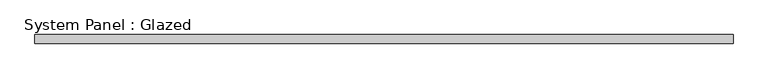
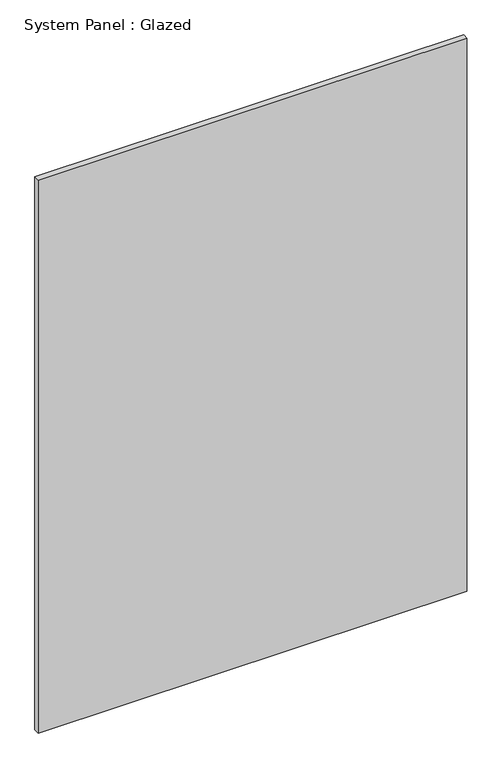
"""IFC4 building model written with IfcOpenShell, lengths in millimetres: plate geometry, System Panel : Glazed."""

from ifc_helpers import new_model, si_unit, origin, origin_with_axes, place, context, project, spatial, polyline, outline, extrude, source, transform, mapped, element, save


def system_panel_glazed_43d21894(model_context):
    return source(origin(), model_context, "Body", "SweptSolid", [
        extrude(outline(polyline([(962.5000001, 24.5), (-962.5000001, 24.5), (-962.5000001, 49.5), (962.5000001, 49.5), (962.5000001, 24.5)])), origin_with_axes(), (0.0, 0.0, 1.0), 2625.0),
    ])


if __name__ == "__main__":
    model = new_model("IFC4")
    model_context = context("Model", 3, world=origin())
    ifc_project = project(units=[si_unit("LENGTHUNIT", "METRE", prefix="MILLI")], contexts=[model_context])
    site = spatial("IfcSite", under=ifc_project)
    building = spatial("IfcBuilding", under=site)
    placement = place(None, origin())
    system_panel_glazed_shape = system_panel_glazed_43d21894(model_context)
    element("IfcPlate", 1, ObjectType="System Panel : Glazed", at=placement, inside=building, context=model_context, shape_type="MappedRepresentation", body=[
        mapped(system_panel_glazed_shape, transform((0.0, 0.0, 0.0), x_axis=(1.0, 0.0, 0.0), y_axis=(0.0, 1.0, 0.0), z_axis=(0.0, 0.0, 1.0))),
    ])
    save(model, "model.ifc")

# Revit data of these elements
# Element 1 (IfcPlate, "System Panel : Glazed")
#   Materials on its faces: "Glass"
# Materials
#   "Glass": class "Glass", colour RGB 0 128 192, transparency 0.9
